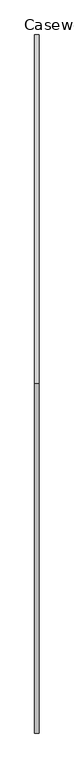
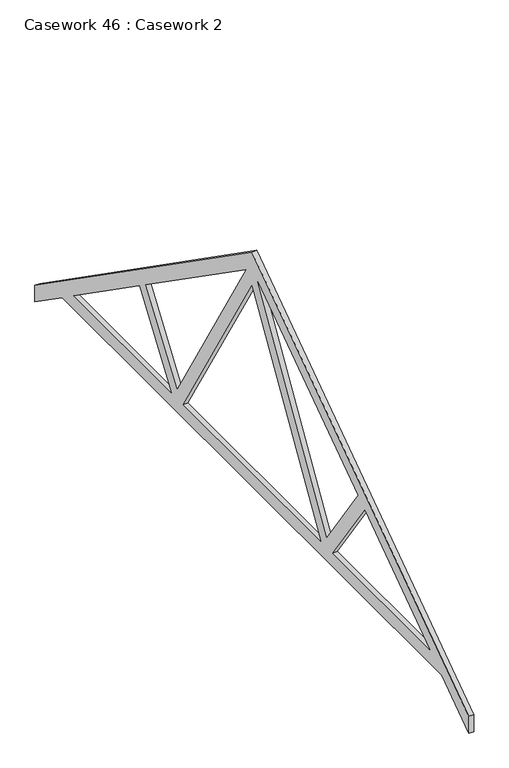
"""IFC4 building model written with IfcOpenShell, lengths in millimetres: furniture geometry, Casework 46 : Casework 2."""

from ifc_helpers import new_model, si_unit, frame, origin, place, context, project, spatial, polyline, outline, extrude, source, transform, mapped, element, save


def casework_46_casework_2_9ef60b2c(model_context):
    return source(origin(), model_context, "Body", "SweptSolid", [
        extrude(outline(polyline([(6583.1149316, 5250.0), (-277.3850684, 5250.0), (-767.3850684, 4906.8983063), (-767.3850684, 5090.0144946), (3152.8649316, 7835.0030963), (7073.1149316, 5090.0144946), (7073.1149316, 4906.8983063), (6583.1149316, 5250.0)]), holes=[polyline([(4612.3149663, 5400.0), (6368.8927306, 5400.0), (5190.2113591, 6225.3215815), (4612.3149663, 5400.0)]), polyline([(4394.2037684, 5400.0), (3152.8649316, 7465.9347567), (1911.5260948, 5400.0), (4394.2037684, 5400.0)]), polyline([(4504.5438357, 5507.6038939), (5067.3385525, 6311.3580469), (3262.0771677, 7575.415677), (4504.5438357, 5507.6038939)]), polyline([(1693.4148969, 5400.0), (1115.5185041, 6225.3215815), (-63.1628674, 5400.0), (1693.4148969, 5400.0)]), polyline([(1801.1860276, 5507.6038939), (3043.6526956, 7575.415677), (1238.3913108, 6311.3580469), (1801.1860276, 5507.6038939)])]), frame((-10421.5247381, 0.0, 0.0), z_axis=(1.0, 0.0, 0.0), x_axis=(0.0, 1.0, 0.0)), (0.0, 0.0, 1.0), 49.6351915),
    ])


if __name__ == "__main__":
    model = new_model("IFC4")
    model_context = context("Model", 3, world=origin())
    ifc_project = project(units=[si_unit("LENGTHUNIT", "METRE", prefix="MILLI")], contexts=[model_context])
    site = spatial("IfcSite", under=ifc_project)
    building = spatial("IfcBuilding", under=site)
    placement = place(None, origin())
    casework_46_casework_2_shape = casework_46_casework_2_9ef60b2c(model_context)
    element("IfcFurniture", 1, ObjectType="Casework 46 : Casework 2", at=placement, inside=building, context=model_context, shape_type="MappedRepresentation", body=[
        mapped(casework_46_casework_2_shape, transform((0.0, 0.0, 0.0), x_axis=(1.0, 0.0, 0.0), y_axis=(0.0, 1.0, 0.0), z_axis=(0.0, 0.0, 1.0))),
    ])
    save(model, "model.ifc")

# Revit data of these elements
# Type "Casework 46 : Casework 2"
#   Manufacturer = "M W Roofs"
#   Type Comments = "Gangnail Roof Truss"
#   Finish = "Rough"
#   Construction Type = "Timber"
# Element 1 (IfcFurniture, "Casework 46 : Casework 2")
#   Materials on its faces: "Softwood, Lumber"
# Materials
#   "Softwood, Lumber": class "Wood", colour RGB 205 156 65, transparency 0, Description = "Pinus Echinata", Cost = 0
